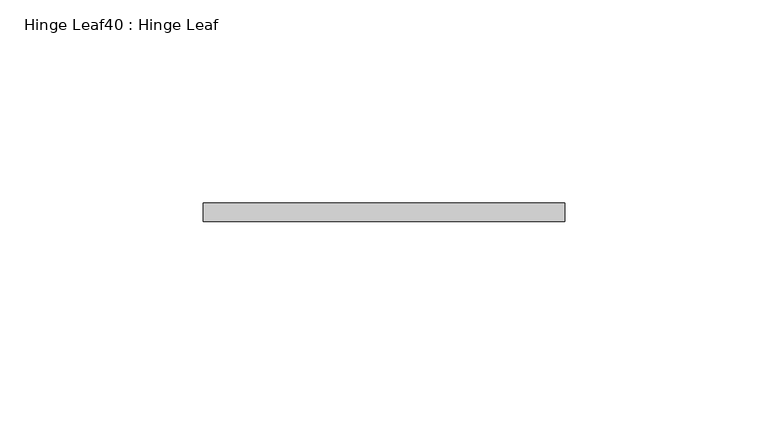
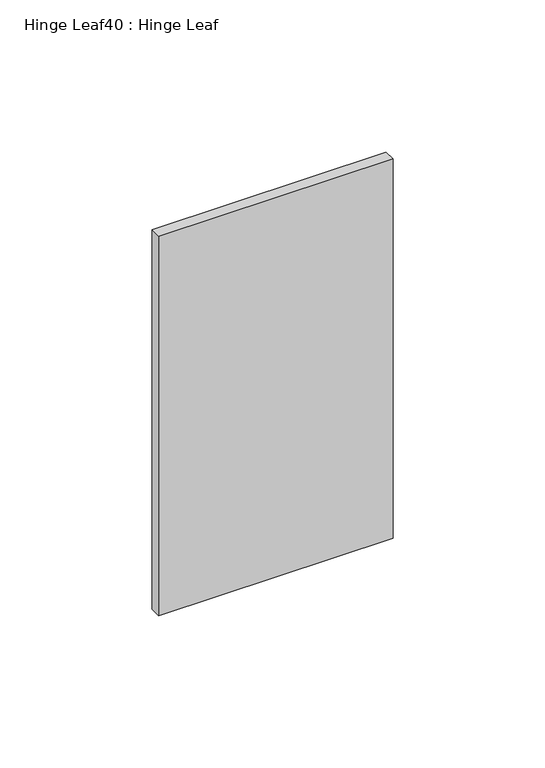
"""IFC4 building model written with IfcOpenShell, lengths in millimetres: proxy geometry, Hinge Leaf40 : Hinge Leaf."""

import ifcopenshell
import ifcopenshell.guid

model = None  # the IFC model being written
_history = None  # IfcOwnerHistory: only IFC2X3 demands one
_inside = {}  # id of a spatial element -> (the spatial element, [elements in it])
_under = {}  # id of a project, library or spatial element -> (it, [spatial elements below it])
_declared = {}  # id of a project -> (the project, [libraries it declares])
_typed = {}  # id of a type object -> (the type object, [elements of that type])
_made_of = {}  # id of a material, layer set ... -> (it, [elements and type objects made of it])


def new_model(schema):
    """Start an empty IFC model of exactly this schema.

    Asked for "IFC4X3", IfcOpenShell would pick the latest addendum, in which some entities
    have other attributes; the version numbers below select the first issue.
    IFC2X3 requires an IfcOwnerHistory on every rooted entity: one is made here for all.
    """
    global model, _history
    if schema == "IFC4X3":
        model = ifcopenshell.file(schema_version=(4, 3, 0, 0))
    else:
        model = ifcopenshell.file(schema=schema)
    _inside.clear()
    _under.clear()
    _declared.clear()
    _typed.clear()
    _made_of.clear()
    _history = None
    if model.schema == "IFC2X3":
        org = make("IfcOrganization", Name="unknown")
        user = make(
            "IfcPersonAndOrganization",
            ThePerson=make("IfcPerson", FamilyName="unknown"),
            TheOrganization=org,
        )
        app = make(
            "IfcApplication",
            ApplicationDeveloper=org,
            Version="unknown",
            ApplicationFullName="unknown",
            ApplicationIdentifier="unknown",
        )
        _history = make(
            "IfcOwnerHistory",
            OwningUser=user,
            OwningApplication=app,
            ChangeAction="ADDED",
            CreationDate=0,
        )
    return model


def make(cls, **values):
    """One entity of the class cls with the attributes given. An attribute that is None is left unset."""
    return model.create_entity(
        cls, **{name: value for name, value in values.items() if value is not None}
    )


def rooted(cls, **values):
    """An entity with a GlobalId (a new one), such as an element, a storey or a relation."""
    return make(cls, GlobalId=ifcopenshell.guid.new(), OwnerHistory=_history, **values)


def si_unit(unit_type, name, prefix=None):
    """IfcSIUnit, for example si_unit("LENGTHUNIT", "METRE", prefix="MILLI")."""
    return make("IfcSIUnit", UnitType=unit_type, Prefix=prefix, Name=name)


def assignment(units):
    """IfcUnitAssignment: the units of a project."""
    return None if units is None else make("IfcUnitAssignment", Units=units)


def point(xyz):
    """IfcCartesianPoint."""
    return None if xyz is None else make("IfcCartesianPoint", Coordinates=xyz)


def direction(xyz):
    """IfcDirection."""
    return None if xyz is None else make("IfcDirection", DirectionRatios=xyz)


def frame(location, z_axis=None, x_axis=None):
    """IfcAxis2Placement3D, a coordinate frame: its origin and axes. An axis left out is left unset."""
    return make(
        "IfcAxis2Placement3D",
        Location=point(location),
        Axis=direction(z_axis),
        RefDirection=direction(x_axis),
    )


def origin():
    """The frame at (0, 0, 0) with its axes left unset."""
    return frame((0.0, 0.0, 0.0))


def place(relative_to, where):
    """IfcLocalPlacement: puts the frame where relative to a parent placement (None: the world)."""
    return make(
        "IfcLocalPlacement", PlacementRelTo=relative_to, RelativePlacement=where
    )


def context(
    kind, dimensions, precision=None, world=None, true_north=None, identifier=None
):
    """IfcGeometricRepresentationContext, for example the 3D "Model" context."""
    return make(
        "IfcGeometricRepresentationContext",
        ContextIdentifier=identifier,
        ContextType=kind,
        CoordinateSpaceDimension=dimensions,
        Precision=precision,
        WorldCoordinateSystem=world,
        TrueNorth=true_north,
    )


def project(units=None, contexts=None):
    """IfcProject with its units and contexts."""
    return rooted(
        "IfcProject",
        Name="project",
        RepresentationContexts=contexts,
        UnitsInContext=assignment(units),
    )


def spatial(cls, under=None, at=None, **own):
    """A site, building, storey or space (cls), placed at a placement, below another one or the project."""
    s = rooted(cls, ObjectPlacement=at, **own)
    if under is not None:
        _under.setdefault(under.id(), (under, []))[1].append(s)
    return s


def polyline(points):
    """IfcPolyline through the points."""
    return make("IfcPolyline", Points=[point(p) for p in points])


def outline(outer, holes=None, kind="AREA"):
    """IfcArbitraryClosedProfileDef: a profile drawn as a closed curve; with holes, ...WithVoids."""
    if holes is None:
        return make("IfcArbitraryClosedProfileDef", ProfileType=kind, OuterCurve=outer)
    return make(
        "IfcArbitraryProfileDefWithVoids",
        ProfileType=kind,
        OuterCurve=outer,
        InnerCurves=holes,
    )


def extrude(swept, where, along, depth):
    """IfcExtrudedAreaSolid: the profile swept, set in the frame where, extruded along a direction by depth."""
    return make(
        "IfcExtrudedAreaSolid",
        SweptArea=swept,
        Position=where,
        ExtrudedDirection=direction(along),
        Depth=depth,
    )


def shape(context_of_items, identifier, shape_type, items):
    """IfcShapeRepresentation: the items that make up one representation, for example the "Body"."""
    return make(
        "IfcShapeRepresentation",
        ContextOfItems=context_of_items,
        RepresentationIdentifier=identifier,
        RepresentationType=shape_type,
        Items=items,
    )


def source(mapping_origin, context_of_items, identifier, shape_type, items):
    """IfcRepresentationMap: a shape defined once, which mapped items show again and again."""
    return make(
        "IfcRepresentationMap",
        MappingOrigin=mapping_origin,
        MappedRepresentation=shape(context_of_items, identifier, shape_type, items),
    )


def transform(
    local_origin,
    x_axis=None,
    y_axis=None,
    z_axis=None,
    scale=None,
    scale2=None,
    scale3=None,
    uniform=True,
):
    """IfcCartesianTransformationOperator3D, or its non-uniform kind. x_axis, y_axis, z_axis: its Axis1, 2, 3."""
    if uniform:
        return make(
            "IfcCartesianTransformationOperator3D",
            Axis1=direction(x_axis),
            Axis2=direction(y_axis),
            LocalOrigin=point(local_origin),
            Scale=scale,
            Axis3=direction(z_axis),
        )
    return make(
        "IfcCartesianTransformationOperator3DnonUniform",
        Axis1=direction(x_axis),
        Axis2=direction(y_axis),
        LocalOrigin=point(local_origin),
        Scale=scale,
        Axis3=direction(z_axis),
        Scale2=scale2,
        Scale3=scale3,
    )


def mapped(mapping_source, mapping_target):
    """IfcMappedItem: shows the shape of a source again, moved by a transform."""
    return make(
        "IfcMappedItem", MappingSource=mapping_source, MappingTarget=mapping_target
    )


def made_of(thing, what):
    """Note that an element or type object is made of a material, layer set ...; save() writes the relation."""
    if what is not None:
        _made_of.setdefault(what.id(), (what, []))[1].append(thing)
    return thing


def element(
    cls,
    number,
    at=None,
    inside=None,
    cuts=None,
    type_object=None,
    material=None,
    context=None,
    identifier="Body",
    shape_type=None,
    held_by="IfcProductDefinitionShape",
    body=None,
    shapes=None,
    **own,
):
    """One element of the class cls, such as IfcWall. Its Tag is "e" and its number.

    at: its placement. inside: the storey or other place that contains it. cuts: it is an
    opening in that element (IfcRelVoidsElement). A single representation is given by context,
    identifier, shape_type and body (its items); several are given by shapes. held_by: the class
    of the entity that holds the representations. save() writes the other relations.
    """
    e = rooted(cls, Tag="e%d" % number, ObjectPlacement=at, **own)
    if body is not None:
        shapes = [shape(context, identifier, shape_type, body)]
    if shapes is not None:
        e.Representation = make(held_by, Representations=shapes)
    if inside is not None:
        _inside.setdefault(inside.id(), (inside, []))[1].append(e)
    if cuts is not None:
        rooted(
            "IfcRelVoidsElement", RelatingBuildingElement=cuts, RelatedOpeningElement=e
        )
    if type_object is not None:
        _typed.setdefault(type_object.id(), (type_object, []))[1].append(e)
    return made_of(e, material)


def aggregate(whole, parts):
    """IfcRelAggregates: a whole, such as a stair, and the parts it consists of."""
    return rooted("IfcRelAggregates", RelatingObject=whole, RelatedObjects=parts)


def save(model, path):
    """Write the relations noted so far, then the file.

    IfcRelAggregates (storeys below a building ...), IfcRelContainedInSpatialStructure (elements
    in a storey), IfcRelDefinesByType, IfcRelAssociatesMaterial and IfcRelDeclares: one each for
    every whole, place, type object, material and project.
    """
    for whole, parts in _under.values():
        aggregate(whole, parts)
    for where, things in _inside.values():
        rooted(
            "IfcRelContainedInSpatialStructure",
            RelatedElements=things,
            RelatingStructure=where,
        )
    for kind, things in _typed.values():
        rooted("IfcRelDefinesByType", RelatedObjects=things, RelatingType=kind)
    for what, things in _made_of.values():
        rooted("IfcRelAssociatesMaterial", RelatedObjects=things, RelatingMaterial=what)
    for by, libraries in _declared.values():
        rooted("IfcRelDeclares", RelatingContext=by, RelatedDefinitions=libraries)
    model.write(path)


def hinge_leaf40_hinge_leaf_89afeb32(model_context):
    return source(origin(), model_context, "Body", "SweptSolid", [
        extrude(outline(polyline([(587327.7934739, -534104.7943841), (587416.6934739, -534104.7943841), (587416.6934739, -534109.3663841), (587327.7934739, -534109.3663841), (587327.7934739, -534104.7943841)])), frame((0.0, 0.0, 1936.75), z_axis=(0.0, 0.0, 1.0), x_axis=(1.0, 0.0, 0.0)), (0.0, 0.0, 1.0), 152.4),
    ])


if __name__ == "__main__":
    model = new_model("IFC4")
    model_context = context("Model", 3, world=origin())
    ifc_project = project(units=[si_unit("LENGTHUNIT", "METRE", prefix="MILLI")], contexts=[model_context])
    site = spatial("IfcSite", under=ifc_project)
    building = spatial("IfcBuilding", under=site)
    placement = place(None, origin())
    hinge_leaf40_hinge_leaf_shape = hinge_leaf40_hinge_leaf_89afeb32(model_context)
    element("IfcBuildingElementProxy", 1, Name="Hinge Leaf40 : Hinge Leaf", ObjectType="Hinge Leaf40 : Hinge Leaf", at=placement, inside=building, context=model_context, shape_type="MappedRepresentation", body=[
        mapped(hinge_leaf40_hinge_leaf_shape, transform((0.0, 0.0, 0.0), x_axis=(1.0, 0.0, 0.0), y_axis=(0.0, 1.0, 0.0), z_axis=(0.0, 0.0, 1.0))),
    ])
    save(model, "model.ifc")

# Revit data of these elements
# Element 1 (IfcBuildingElementProxy, "Hinge Leaf40 : Hinge Leaf")
#   Materials on its faces: "6\"X6\" WELD-ON STL BUTT HINGE"
# Materials
#   "6\"X6\" WELD-ON STL BUTT HINGE": class "Metal", colour RGB 189 187 185, transparency 0, Description = "Carbon steel", Cost = 0
